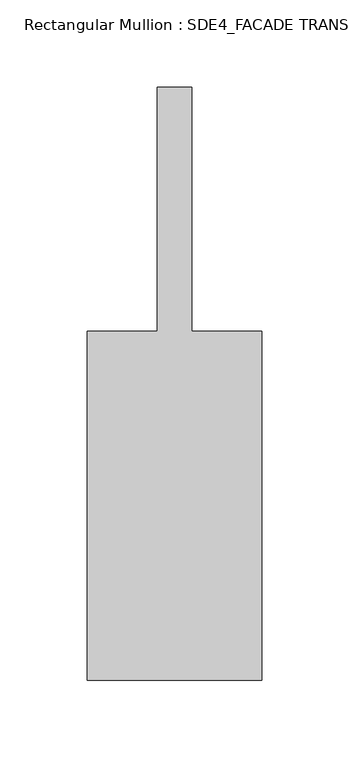
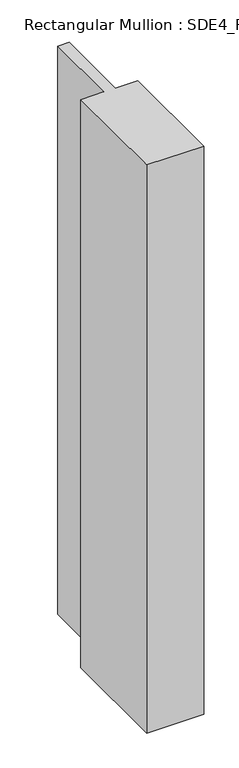
"""IFC4 building model written with IfcOpenShell, lengths in millimetres: member geometry, Rectangular Mullion : SDE4_FACADE TRANSOM TYPE 1."""

import ifcopenshell
import ifcopenshell.guid

model = None  # the IFC model being written
_history = None  # IfcOwnerHistory: only IFC2X3 demands one
_inside = {}  # id of a spatial element -> (the spatial element, [elements in it])
_under = {}  # id of a project, library or spatial element -> (it, [spatial elements below it])
_declared = {}  # id of a project -> (the project, [libraries it declares])
_typed = {}  # id of a type object -> (the type object, [elements of that type])
_made_of = {}  # id of a material, layer set ... -> (it, [elements and type objects made of it])


def new_model(schema):
    """Start an empty IFC model of exactly this schema.

    Asked for "IFC4X3", IfcOpenShell would pick the latest addendum, in which some entities
    have other attributes; the version numbers below select the first issue.
    IFC2X3 requires an IfcOwnerHistory on every rooted entity: one is made here for all.
    """
    global model, _history
    if schema == "IFC4X3":
        model = ifcopenshell.file(schema_version=(4, 3, 0, 0))
    else:
        model = ifcopenshell.file(schema=schema)
    _inside.clear()
    _under.clear()
    _declared.clear()
    _typed.clear()
    _made_of.clear()
    _history = None
    if model.schema == "IFC2X3":
        org = make("IfcOrganization", Name="unknown")
        user = make(
            "IfcPersonAndOrganization",
            ThePerson=make("IfcPerson", FamilyName="unknown"),
            TheOrganization=org,
        )
        app = make(
            "IfcApplication",
            ApplicationDeveloper=org,
            Version="unknown",
            ApplicationFullName="unknown",
            ApplicationIdentifier="unknown",
        )
        _history = make(
            "IfcOwnerHistory",
            OwningUser=user,
            OwningApplication=app,
            ChangeAction="ADDED",
            CreationDate=0,
        )
    return model


def make(cls, **values):
    """One entity of the class cls with the attributes given. An attribute that is None is left unset."""
    return model.create_entity(
        cls, **{name: value for name, value in values.items() if value is not None}
    )


def rooted(cls, **values):
    """An entity with a GlobalId (a new one), such as an element, a storey or a relation."""
    return make(cls, GlobalId=ifcopenshell.guid.new(), OwnerHistory=_history, **values)


def si_unit(unit_type, name, prefix=None):
    """IfcSIUnit, for example si_unit("LENGTHUNIT", "METRE", prefix="MILLI")."""
    return make("IfcSIUnit", UnitType=unit_type, Prefix=prefix, Name=name)


def assignment(units):
    """IfcUnitAssignment: the units of a project."""
    return None if units is None else make("IfcUnitAssignment", Units=units)


def point(xyz):
    """IfcCartesianPoint."""
    return None if xyz is None else make("IfcCartesianPoint", Coordinates=xyz)


def direction(xyz):
    """IfcDirection."""
    return None if xyz is None else make("IfcDirection", DirectionRatios=xyz)


def frame(location, z_axis=None, x_axis=None):
    """IfcAxis2Placement3D, a coordinate frame: its origin and axes. An axis left out is left unset."""
    return make(
        "IfcAxis2Placement3D",
        Location=point(location),
        Axis=direction(z_axis),
        RefDirection=direction(x_axis),
    )


def origin():
    """The frame at (0, 0, 0) with its axes left unset."""
    return frame((0.0, 0.0, 0.0))


def place(relative_to, where):
    """IfcLocalPlacement: puts the frame where relative to a parent placement (None: the world)."""
    return make(
        "IfcLocalPlacement", PlacementRelTo=relative_to, RelativePlacement=where
    )


def context(
    kind, dimensions, precision=None, world=None, true_north=None, identifier=None
):
    """IfcGeometricRepresentationContext, for example the 3D "Model" context."""
    return make(
        "IfcGeometricRepresentationContext",
        ContextIdentifier=identifier,
        ContextType=kind,
        CoordinateSpaceDimension=dimensions,
        Precision=precision,
        WorldCoordinateSystem=world,
        TrueNorth=true_north,
    )


def project(units=None, contexts=None):
    """IfcProject with its units and contexts."""
    return rooted(
        "IfcProject",
        Name="project",
        RepresentationContexts=contexts,
        UnitsInContext=assignment(units),
    )


def spatial(cls, under=None, at=None, **own):
    """A site, building, storey or space (cls), placed at a placement, below another one or the project."""
    s = rooted(cls, ObjectPlacement=at, **own)
    if under is not None:
        _under.setdefault(under.id(), (under, []))[1].append(s)
    return s


def polyline(points):
    """IfcPolyline through the points."""
    return make("IfcPolyline", Points=[point(p) for p in points])


def outline(outer, holes=None, kind="AREA"):
    """IfcArbitraryClosedProfileDef: a profile drawn as a closed curve; with holes, ...WithVoids."""
    if holes is None:
        return make("IfcArbitraryClosedProfileDef", ProfileType=kind, OuterCurve=outer)
    return make(
        "IfcArbitraryProfileDefWithVoids",
        ProfileType=kind,
        OuterCurve=outer,
        InnerCurves=holes,
    )


def extrude(swept, where, along, depth):
    """IfcExtrudedAreaSolid: the profile swept, set in the frame where, extruded along a direction by depth."""
    return make(
        "IfcExtrudedAreaSolid",
        SweptArea=swept,
        Position=where,
        ExtrudedDirection=direction(along),
        Depth=depth,
    )


def shape(context_of_items, identifier, shape_type, items):
    """IfcShapeRepresentation: the items that make up one representation, for example the "Body"."""
    return make(
        "IfcShapeRepresentation",
        ContextOfItems=context_of_items,
        RepresentationIdentifier=identifier,
        RepresentationType=shape_type,
        Items=items,
    )


def source(mapping_origin, context_of_items, identifier, shape_type, items):
    """IfcRepresentationMap: a shape defined once, which mapped items show again and again."""
    return make(
        "IfcRepresentationMap",
        MappingOrigin=mapping_origin,
        MappedRepresentation=shape(context_of_items, identifier, shape_type, items),
    )


def transform(
    local_origin,
    x_axis=None,
    y_axis=None,
    z_axis=None,
    scale=None,
    scale2=None,
    scale3=None,
    uniform=True,
):
    """IfcCartesianTransformationOperator3D, or its non-uniform kind. x_axis, y_axis, z_axis: its Axis1, 2, 3."""
    if uniform:
        return make(
            "IfcCartesianTransformationOperator3D",
            Axis1=direction(x_axis),
            Axis2=direction(y_axis),
            LocalOrigin=point(local_origin),
            Scale=scale,
            Axis3=direction(z_axis),
        )
    return make(
        "IfcCartesianTransformationOperator3DnonUniform",
        Axis1=direction(x_axis),
        Axis2=direction(y_axis),
        LocalOrigin=point(local_origin),
        Scale=scale,
        Axis3=direction(z_axis),
        Scale2=scale2,
        Scale3=scale3,
    )


def mapped(mapping_source, mapping_target):
    """IfcMappedItem: shows the shape of a source again, moved by a transform."""
    return make(
        "IfcMappedItem", MappingSource=mapping_source, MappingTarget=mapping_target
    )


def made_of(thing, what):
    """Note that an element or type object is made of a material, layer set ...; save() writes the relation."""
    if what is not None:
        _made_of.setdefault(what.id(), (what, []))[1].append(thing)
    return thing


def element(
    cls,
    number,
    at=None,
    inside=None,
    cuts=None,
    type_object=None,
    material=None,
    context=None,
    identifier="Body",
    shape_type=None,
    held_by="IfcProductDefinitionShape",
    body=None,
    shapes=None,
    **own,
):
    """One element of the class cls, such as IfcWall. Its Tag is "e" and its number.

    at: its placement. inside: the storey or other place that contains it. cuts: it is an
    opening in that element (IfcRelVoidsElement). A single representation is given by context,
    identifier, shape_type and body (its items); several are given by shapes. held_by: the class
    of the entity that holds the representations. save() writes the other relations.
    """
    e = rooted(cls, Tag="e%d" % number, ObjectPlacement=at, **own)
    if body is not None:
        shapes = [shape(context, identifier, shape_type, body)]
    if shapes is not None:
        e.Representation = make(held_by, Representations=shapes)
    if inside is not None:
        _inside.setdefault(inside.id(), (inside, []))[1].append(e)
    if cuts is not None:
        rooted(
            "IfcRelVoidsElement", RelatingBuildingElement=cuts, RelatedOpeningElement=e
        )
    if type_object is not None:
        _typed.setdefault(type_object.id(), (type_object, []))[1].append(e)
    return made_of(e, material)


def aggregate(whole, parts):
    """IfcRelAggregates: a whole, such as a stair, and the parts it consists of."""
    return rooted("IfcRelAggregates", RelatingObject=whole, RelatedObjects=parts)


def save(model, path):
    """Write the relations noted so far, then the file.

    IfcRelAggregates (storeys below a building ...), IfcRelContainedInSpatialStructure (elements
    in a storey), IfcRelDefinesByType, IfcRelAssociatesMaterial and IfcRelDeclares: one each for
    every whole, place, type object, material and project.
    """
    for whole, parts in _under.values():
        aggregate(whole, parts)
    for where, things in _inside.values():
        rooted(
            "IfcRelContainedInSpatialStructure",
            RelatedElements=things,
            RelatingStructure=where,
        )
    for kind, things in _typed.values():
        rooted("IfcRelDefinesByType", RelatedObjects=things, RelatingType=kind)
    for what, things in _made_of.values():
        rooted("IfcRelAssociatesMaterial", RelatedObjects=things, RelatingMaterial=what)
    for by, libraries in _declared.values():
        rooted("IfcRelDeclares", RelatingContext=by, RelatedDefinitions=libraries)
    model.write(path)


def rectangular_mullion_sde4_facade_transom_type_1_ee32d7e8(model_context):
    return source(origin(), model_context, "Body", "SweptSolid", [
        extrude(outline(polyline([(50.0, -132.5), (-50.0, -132.5), (-50.0, 67.5), (-10.0, 67.5), (-10.0, 207.5), (10.0, 207.5), (10.0, 67.5), (50.0, 67.5), (50.0, -132.5)])), frame((0.0, 0.0, -1054.0), z_axis=(0.0, 0.0, 1.0), x_axis=(1.0, 0.0, 0.0)), (0.0, 0.0, 1.0), 1054.0),
    ])


if __name__ == "__main__":
    model = new_model("IFC4")
    model_context = context("Model", 3, world=origin())
    ifc_project = project(units=[si_unit("LENGTHUNIT", "METRE", prefix="MILLI")], contexts=[model_context])
    site = spatial("IfcSite", under=ifc_project)
    building = spatial("IfcBuilding", under=site)
    placement = place(None, origin())
    rectangular_mullion_sde4_facade_transom_type_1_shape = rectangular_mullion_sde4_facade_transom_type_1_ee32d7e8(model_context)
    element("IfcMember", 1, ObjectType="Rectangular Mullion : SDE4_FACADE TRANSOM TYPE 1", at=placement, inside=building, context=model_context, shape_type="MappedRepresentation", body=[
        mapped(rectangular_mullion_sde4_facade_transom_type_1_shape, transform((0.0, 0.0, 0.0), x_axis=(1.0, 0.0, 0.0), y_axis=(0.0, 1.0, 0.0), z_axis=(0.0, 0.0, 1.0))),
    ])
    save(model, "model.ifc")

# Revit data of these elements
# Type "Rectangular Mullion : SDE4_FACADE TRANSOM TYPE 1"
#   built-in parameter 1007322 = 1.11549 (stored number, unit not read)
#   built-in parameter 1007321 = 0.164042 (stored number, unit not read)
#   built-in parameter 1007320 = 0.164042 (stored number, unit not read)
